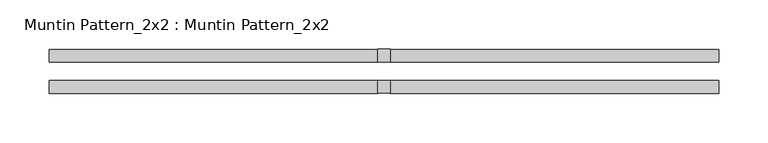
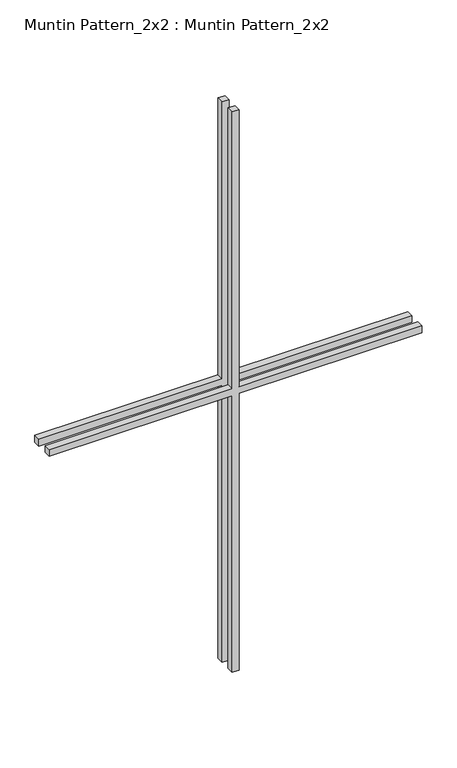
"""IFC4 building model written with IfcOpenShell, lengths in millimetres: proxy geometry, Muntin Pattern_2x2 : Muntin Pattern_2x2."""

import ifcopenshell
import ifcopenshell.guid

model = None  # the IFC model being written
_history = None  # IfcOwnerHistory: only IFC2X3 demands one
_inside = {}  # id of a spatial element -> (the spatial element, [elements in it])
_under = {}  # id of a project, library or spatial element -> (it, [spatial elements below it])
_declared = {}  # id of a project -> (the project, [libraries it declares])
_typed = {}  # id of a type object -> (the type object, [elements of that type])
_made_of = {}  # id of a material, layer set ... -> (it, [elements and type objects made of it])


def new_model(schema):
    """Start an empty IFC model of exactly this schema.

    Asked for "IFC4X3", IfcOpenShell would pick the latest addendum, in which some entities
    have other attributes; the version numbers below select the first issue.
    IFC2X3 requires an IfcOwnerHistory on every rooted entity: one is made here for all.
    """
    global model, _history
    if schema == "IFC4X3":
        model = ifcopenshell.file(schema_version=(4, 3, 0, 0))
    else:
        model = ifcopenshell.file(schema=schema)
    _inside.clear()
    _under.clear()
    _declared.clear()
    _typed.clear()
    _made_of.clear()
    _history = None
    if model.schema == "IFC2X3":
        org = make("IfcOrganization", Name="unknown")
        user = make(
            "IfcPersonAndOrganization",
            ThePerson=make("IfcPerson", FamilyName="unknown"),
            TheOrganization=org,
        )
        app = make(
            "IfcApplication",
            ApplicationDeveloper=org,
            Version="unknown",
            ApplicationFullName="unknown",
            ApplicationIdentifier="unknown",
        )
        _history = make(
            "IfcOwnerHistory",
            OwningUser=user,
            OwningApplication=app,
            ChangeAction="ADDED",
            CreationDate=0,
        )
    return model


def make(cls, **values):
    """One entity of the class cls with the attributes given. An attribute that is None is left unset."""
    return model.create_entity(
        cls, **{name: value for name, value in values.items() if value is not None}
    )


def rooted(cls, **values):
    """An entity with a GlobalId (a new one), such as an element, a storey or a relation."""
    return make(cls, GlobalId=ifcopenshell.guid.new(), OwnerHistory=_history, **values)


def si_unit(unit_type, name, prefix=None):
    """IfcSIUnit, for example si_unit("LENGTHUNIT", "METRE", prefix="MILLI")."""
    return make("IfcSIUnit", UnitType=unit_type, Prefix=prefix, Name=name)


def assignment(units):
    """IfcUnitAssignment: the units of a project."""
    return None if units is None else make("IfcUnitAssignment", Units=units)


def point(xyz):
    """IfcCartesianPoint."""
    return None if xyz is None else make("IfcCartesianPoint", Coordinates=xyz)


def direction(xyz):
    """IfcDirection."""
    return None if xyz is None else make("IfcDirection", DirectionRatios=xyz)


def frame(location, z_axis=None, x_axis=None):
    """IfcAxis2Placement3D, a coordinate frame: its origin and axes. An axis left out is left unset."""
    return make(
        "IfcAxis2Placement3D",
        Location=point(location),
        Axis=direction(z_axis),
        RefDirection=direction(x_axis),
    )


def origin():
    """The frame at (0, 0, 0) with its axes left unset."""
    return frame((0.0, 0.0, 0.0))


def place(relative_to, where):
    """IfcLocalPlacement: puts the frame where relative to a parent placement (None: the world)."""
    return make(
        "IfcLocalPlacement", PlacementRelTo=relative_to, RelativePlacement=where
    )


def context(
    kind, dimensions, precision=None, world=None, true_north=None, identifier=None
):
    """IfcGeometricRepresentationContext, for example the 3D "Model" context."""
    return make(
        "IfcGeometricRepresentationContext",
        ContextIdentifier=identifier,
        ContextType=kind,
        CoordinateSpaceDimension=dimensions,
        Precision=precision,
        WorldCoordinateSystem=world,
        TrueNorth=true_north,
    )


def project(units=None, contexts=None):
    """IfcProject with its units and contexts."""
    return rooted(
        "IfcProject",
        Name="project",
        RepresentationContexts=contexts,
        UnitsInContext=assignment(units),
    )


def spatial(cls, under=None, at=None, **own):
    """A site, building, storey or space (cls), placed at a placement, below another one or the project."""
    s = rooted(cls, ObjectPlacement=at, **own)
    if under is not None:
        _under.setdefault(under.id(), (under, []))[1].append(s)
    return s


def polyline(points):
    """IfcPolyline through the points."""
    return make("IfcPolyline", Points=[point(p) for p in points])


def outline(outer, holes=None, kind="AREA"):
    """IfcArbitraryClosedProfileDef: a profile drawn as a closed curve; with holes, ...WithVoids."""
    if holes is None:
        return make("IfcArbitraryClosedProfileDef", ProfileType=kind, OuterCurve=outer)
    return make(
        "IfcArbitraryProfileDefWithVoids",
        ProfileType=kind,
        OuterCurve=outer,
        InnerCurves=holes,
    )


def extrude(swept, where, along, depth):
    """IfcExtrudedAreaSolid: the profile swept, set in the frame where, extruded along a direction by depth."""
    return make(
        "IfcExtrudedAreaSolid",
        SweptArea=swept,
        Position=where,
        ExtrudedDirection=direction(along),
        Depth=depth,
    )


def shape(context_of_items, identifier, shape_type, items):
    """IfcShapeRepresentation: the items that make up one representation, for example the "Body"."""
    return make(
        "IfcShapeRepresentation",
        ContextOfItems=context_of_items,
        RepresentationIdentifier=identifier,
        RepresentationType=shape_type,
        Items=items,
    )


def source(mapping_origin, context_of_items, identifier, shape_type, items):
    """IfcRepresentationMap: a shape defined once, which mapped items show again and again."""
    return make(
        "IfcRepresentationMap",
        MappingOrigin=mapping_origin,
        MappedRepresentation=shape(context_of_items, identifier, shape_type, items),
    )


def transform(
    local_origin,
    x_axis=None,
    y_axis=None,
    z_axis=None,
    scale=None,
    scale2=None,
    scale3=None,
    uniform=True,
):
    """IfcCartesianTransformationOperator3D, or its non-uniform kind. x_axis, y_axis, z_axis: its Axis1, 2, 3."""
    if uniform:
        return make(
            "IfcCartesianTransformationOperator3D",
            Axis1=direction(x_axis),
            Axis2=direction(y_axis),
            LocalOrigin=point(local_origin),
            Scale=scale,
            Axis3=direction(z_axis),
        )
    return make(
        "IfcCartesianTransformationOperator3DnonUniform",
        Axis1=direction(x_axis),
        Axis2=direction(y_axis),
        LocalOrigin=point(local_origin),
        Scale=scale,
        Axis3=direction(z_axis),
        Scale2=scale2,
        Scale3=scale3,
    )


def mapped(mapping_source, mapping_target):
    """IfcMappedItem: shows the shape of a source again, moved by a transform."""
    return make(
        "IfcMappedItem", MappingSource=mapping_source, MappingTarget=mapping_target
    )


def made_of(thing, what):
    """Note that an element or type object is made of a material, layer set ...; save() writes the relation."""
    if what is not None:
        _made_of.setdefault(what.id(), (what, []))[1].append(thing)
    return thing


def element(
    cls,
    number,
    at=None,
    inside=None,
    cuts=None,
    type_object=None,
    material=None,
    context=None,
    identifier="Body",
    shape_type=None,
    held_by="IfcProductDefinitionShape",
    body=None,
    shapes=None,
    **own,
):
    """One element of the class cls, such as IfcWall. Its Tag is "e" and its number.

    at: its placement. inside: the storey or other place that contains it. cuts: it is an
    opening in that element (IfcRelVoidsElement). A single representation is given by context,
    identifier, shape_type and body (its items); several are given by shapes. held_by: the class
    of the entity that holds the representations. save() writes the other relations.
    """
    e = rooted(cls, Tag="e%d" % number, ObjectPlacement=at, **own)
    if body is not None:
        shapes = [shape(context, identifier, shape_type, body)]
    if shapes is not None:
        e.Representation = make(held_by, Representations=shapes)
    if inside is not None:
        _inside.setdefault(inside.id(), (inside, []))[1].append(e)
    if cuts is not None:
        rooted(
            "IfcRelVoidsElement", RelatingBuildingElement=cuts, RelatedOpeningElement=e
        )
    if type_object is not None:
        _typed.setdefault(type_object.id(), (type_object, []))[1].append(e)
    return made_of(e, material)


def aggregate(whole, parts):
    """IfcRelAggregates: a whole, such as a stair, and the parts it consists of."""
    return rooted("IfcRelAggregates", RelatingObject=whole, RelatedObjects=parts)


def save(model, path):
    """Write the relations noted so far, then the file.

    IfcRelAggregates (storeys below a building ...), IfcRelContainedInSpatialStructure (elements
    in a storey), IfcRelDefinesByType, IfcRelAssociatesMaterial and IfcRelDeclares: one each for
    every whole, place, type object, material and project.
    """
    for whole, parts in _under.values():
        aggregate(whole, parts)
    for where, things in _inside.values():
        rooted(
            "IfcRelContainedInSpatialStructure",
            RelatedElements=things,
            RelatingStructure=where,
        )
    for kind, things in _typed.values():
        rooted("IfcRelDefinesByType", RelatedObjects=things, RelatingType=kind)
    for what, things in _made_of.values():
        rooted("IfcRelAssociatesMaterial", RelatedObjects=things, RelatingMaterial=what)
    for by, libraries in _declared.values():
        rooted("IfcRelDeclares", RelatingContext=by, RelatedDefinitions=libraries)
    model.write(path)


def muntin_pattern_2x2_muntin_pattern_2x2_3179e719(model_context):
    return source(origin(), model_context, "Body", "SweptSolid", [
        extrude(outline(polyline([(542.925, -6.35), (542.925, -338.1375), (530.225, -338.1375), (530.225, -6.35), (0.0, -6.35), (0.0, 6.35), (530.225, 6.35), (530.225, 338.1375), (542.925, 338.1375), (542.925, 6.35), (1073.15, 6.35), (1073.15, -6.35), (542.925, -6.35)])), frame((0.0, 9.525, 0.0), z_axis=(0.0, 1.0, 0.0), x_axis=(0.0, 0.0, 1.0)), (0.0, 0.0, 1.0), 12.7),
        extrude(outline(polyline([(542.925, -6.35), (542.925, -338.1375), (530.225, -338.1375), (530.225, -6.35), (0.0, -6.35), (0.0, 6.35), (530.225, 6.35), (530.225, 338.1375), (542.925, 338.1375), (542.925, 6.35), (1073.15, 6.35), (1073.15, -6.35), (542.925, -6.35)])), frame((0.0, -22.225, 0.0), z_axis=(0.0, 1.0, 0.0), x_axis=(0.0, 0.0, 1.0)), (0.0, 0.0, 1.0), 12.7),
    ])


if __name__ == "__main__":
    model = new_model("IFC4")
    model_context = context("Model", 3, world=origin())
    ifc_project = project(units=[si_unit("LENGTHUNIT", "METRE", prefix="MILLI")], contexts=[model_context])
    site = spatial("IfcSite", under=ifc_project)
    building = spatial("IfcBuilding", under=site)
    placement = place(None, origin())
    muntin_pattern_2x2_muntin_pattern_2x2_shape = muntin_pattern_2x2_muntin_pattern_2x2_3179e719(model_context)
    element("IfcBuildingElementProxy", 1, Name="Muntin Pattern_2x2 : Muntin Pattern_2x2", ObjectType="Muntin Pattern_2x2 : Muntin Pattern_2x2", at=placement, inside=building, context=model_context, shape_type="MappedRepresentation", body=[
        mapped(muntin_pattern_2x2_muntin_pattern_2x2_shape, transform((0.0, 0.0, 0.0), x_axis=(1.0, 0.0, 0.0), y_axis=(0.0, 1.0, 0.0), z_axis=(0.0, 0.0, 1.0))),
    ])
    save(model, "model.ifc")

# Revit data of these elements
# Project information
#   Project Issue Date = "Issue Date"
#   Project Status = "Project Status"
#   Client Name = "Owner"
#   Project Address = "Enter address here"
#   Project Name = "Project Name"
#   Project Number = "Project Number"
# Type "Muntin Pattern_2x2 : Muntin Pattern_2x2"
#   Width [instance default] = 4' - 0"
#   Thickness = 0' - 0 1/2"
#   Height [instance default] = 4' - 0"
#   Distance = 0' - 0 3/4"
#   Interior Material [instance default] = none
#   Exterior Material [instance default] = none
#   Default Elevation = 0
# Element 1 (IfcBuildingElementProxy, "Muntin Pattern_2x2 : Muntin Pattern_2x2")
#   Width = 2' - 2 5/8"
#   Height = 3' - 6 1/4"
#   Interior Material = Wood - Stained
#   Exterior Material = Clad - White
#   Materials on its faces: "Clad - White", "Wood - Stained"
# Materials
#   "Clad - White": class "Wood", colour RGB 242 242 238, transparency 0, Cost = 0
#   "Wood - Stained": class "Wood", colour RGB 227 170 128, transparency 0, Cost = 0
